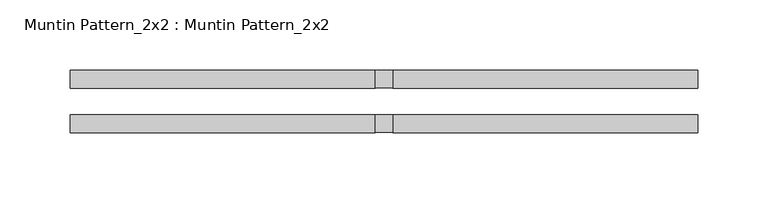
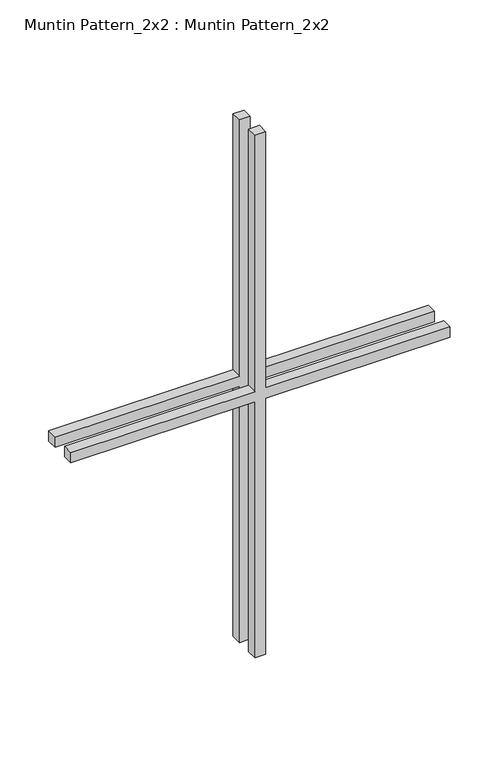
"""IFC4 building model written with IfcOpenShell, lengths in millimetres: proxy geometry, Muntin Pattern_2x2 : Muntin Pattern_2x2."""

from ifc_helpers import new_model, si_unit, frame, origin, place, context, project, spatial, polyline, outline, extrude, source, transform, mapped, element, save


def muntin_pattern_2x2_muntin_pattern_2x2_5bc09aa8(model_context):
    return source(origin(), model_context, "Body", "SweptSolid", [
        extrude(outline(polyline([(332.1375, -6.35), (332.1375, -223.8), (319.4375, -223.8), (319.4375, -6.35), (0.0, -6.35), (0.0, 6.35), (319.4375, 6.35), (319.4375, 223.8), (332.1375, 223.8), (332.1375, 6.35), (651.575, 6.35), (651.575, -6.35), (332.1375, -6.35)])), frame((0.0, 9.525, 0.0), z_axis=(0.0, 1.0, 0.0), x_axis=(0.0, 0.0, 1.0)), (0.0, 0.0, 1.0), 12.7),
        extrude(outline(polyline([(332.1375, -6.35), (332.1375, -223.8), (319.4375, -223.8), (319.4375, -6.35), (0.0, -6.35), (0.0, 6.35), (319.4375, 6.35), (319.4375, 223.8), (332.1375, 223.8), (332.1375, 6.35), (651.575, 6.35), (651.575, -6.35), (332.1375, -6.35)])), frame((0.0, -22.225, 0.0), z_axis=(0.0, 1.0, 0.0), x_axis=(0.0, 0.0, 1.0)), (0.0, 0.0, 1.0), 12.7),
    ])


if __name__ == "__main__":
    model = new_model("IFC4")
    model_context = context("Model", 3, world=origin())
    ifc_project = project(units=[si_unit("LENGTHUNIT", "METRE", prefix="MILLI")], contexts=[model_context])
    site = spatial("IfcSite", under=ifc_project)
    building = spatial("IfcBuilding", under=site)
    placement = place(None, origin())
    muntin_pattern_2x2_muntin_pattern_2x2_shape = muntin_pattern_2x2_muntin_pattern_2x2_5bc09aa8(model_context)
    element("IfcBuildingElementProxy", 1, Name="Muntin Pattern_2x2 : Muntin Pattern_2x2", ObjectType="Muntin Pattern_2x2 : Muntin Pattern_2x2", at=placement, inside=building, context=model_context, shape_type="MappedRepresentation", body=[
        mapped(muntin_pattern_2x2_muntin_pattern_2x2_shape, transform((0.0, 0.0, 0.0), x_axis=(1.0, 0.0, 0.0), y_axis=(0.0, 1.0, 0.0), z_axis=(0.0, 0.0, 1.0))),
    ])
    save(model, "model.ifc")

# Revit data of these elements
# Type "Muntin Pattern_2x2 : Muntin Pattern_2x2"
#   Width [instance default] = 121.92 cm
#   Thickness = 1.27 cm
#   Height [instance default] = 121.92 cm
#   Distance = 1.905 cm
#   Interior Material [instance default] = none
#   Exterior Material [instance default] = none
# Element 1 (IfcBuildingElementProxy, "Muntin Pattern_2x2 : Muntin Pattern_2x2")
#   Width = 44.76 cm
#   Height = 65.1575 cm
#   Interior Material = Wood - Stained
#   Exterior Material = Clad - White
#   Materials on its faces: "Clad - White", "Wood - Stained"
# Materials
#   "Clad - White": class "Wood", colour RGB 242 242 238, transparency 0, Cost = 0
#   "Wood - Stained": class "Wood", colour RGB 224 178 126, transparency 0, Cost = 0
